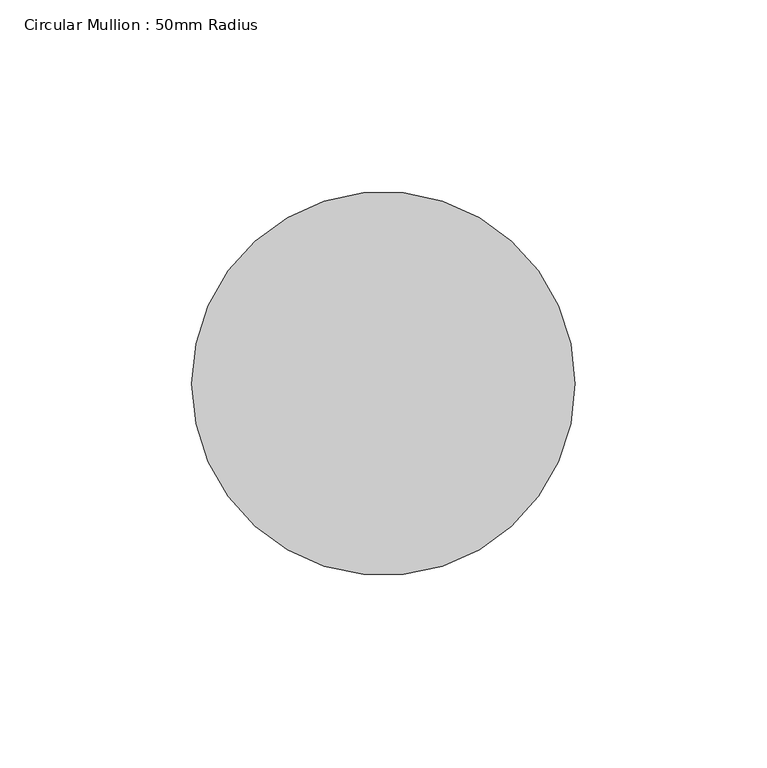
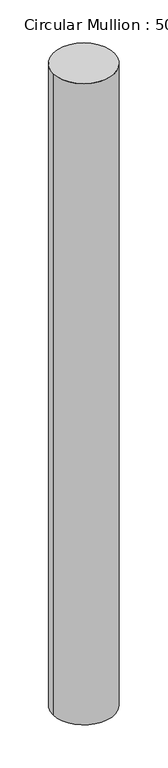
"""IFC4 building model written with IfcOpenShell, lengths in millimetres: member geometry, Circular Mullion : 50mm Radius."""

from ifc_helpers import new_model, si_unit, point, frame, origin, origin_2d, place, context, project, spatial, circle_curve, trimmed, segment, composite_curve, outline, extrude, source, transform, mapped, element, save


def circular_mullion_50mm_radius_9f5787b8(model_context):
    return source(origin(), model_context, "Body", "SweptSolid", [
        extrude(outline(composite_curve([segment(trimmed(circle_curve(origin_2d(), 50.0), [point((50.0, 0.0))], [point((-50.0, 0.0))], False, "CARTESIAN"), True, "CONTINUOUS"), segment(trimmed(circle_curve(origin_2d(), 50.0), [point((-50.0, 0.0))], [point((50.0, 0.0))], False, "CARTESIAN"), True, "CONTINUOUS")], self_intersect=False)), frame((0.0, 0.0, -1101.9269737), z_axis=(0.0, 0.0, 1.0), x_axis=(1.0, 0.0, 0.0)), (0.0, 0.0, 1.0), 1101.9269737),
    ])


if __name__ == "__main__":
    model = new_model("IFC4")
    model_context = context("Model", 3, world=origin())
    ifc_project = project(units=[si_unit("LENGTHUNIT", "METRE", prefix="MILLI")], contexts=[model_context])
    site = spatial("IfcSite", under=ifc_project)
    building = spatial("IfcBuilding", under=site)
    placement = place(None, origin())
    circular_mullion_50mm_radius_shape = circular_mullion_50mm_radius_9f5787b8(model_context)
    element("IfcMember", 1, ObjectType="Circular Mullion : 50mm Radius", at=placement, inside=building, context=model_context, shape_type="MappedRepresentation", body=[
        mapped(circular_mullion_50mm_radius_shape, transform((0.0, 0.0, 0.0), x_axis=(1.0, 0.0, 0.0), y_axis=(0.0, 1.0, 0.0), z_axis=(0.0, 0.0, 1.0))),
    ])
    save(model, "model.ifc")

# Revit data of these elements
# Type "Circular Mullion : 50mm Radius"
#   built-in parameter 1007350 = 0.164042 (stored number, unit not read)
# Element 1 (IfcMember, "Circular Mullion : 50mm Radius")
#   Materials on its faces: "Aluminium"
# Materials
#   "Aluminium": class "Metal", colour RGB 247 247 247, transparency 0, Description = "Aluminium 6061", Cost = 0
